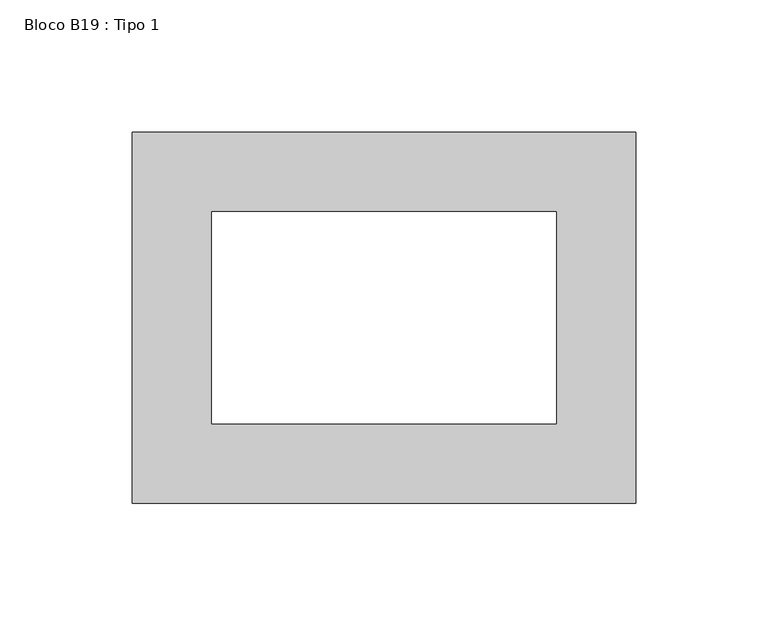
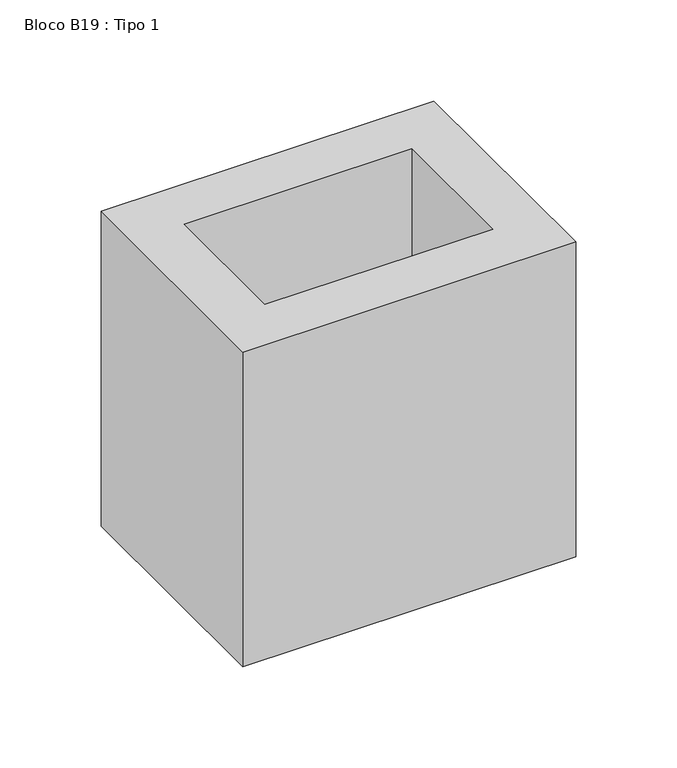
"""IFC4 building model written with IfcOpenShell, lengths in millimetres: proxy geometry, Bloco B19 : Tipo 1."""

from ifc_helpers import new_model, si_unit, origin, origin_with_axes, place, context, project, spatial, polyline, outline, extrude, source, transform, mapped, element, save


def bloco_b19_tipo_1_1abb6ed9(model_context):
    return source(origin(), model_context, "Body", "SweptSolid", [
        extrude(outline(polyline([(190.0, 140.0), (190.0, 0.0), (0.0, 0.0), (0.0, 140.0), (190.0, 140.0)]), holes=[polyline([(30.0, 110.0), (30.0, 30.0), (160.0, 30.0), (160.0, 110.0), (30.0, 110.0)])]), origin_with_axes(), (0.0, 0.0, 1.0), 190.0),
    ])


if __name__ == "__main__":
    model = new_model("IFC4")
    model_context = context("Model", 3, world=origin())
    ifc_project = project(units=[si_unit("LENGTHUNIT", "METRE", prefix="MILLI")], contexts=[model_context])
    site = spatial("IfcSite", under=ifc_project)
    building = spatial("IfcBuilding", under=site)
    placement = place(None, origin())
    bloco_b19_tipo_1_shape = bloco_b19_tipo_1_1abb6ed9(model_context)
    element("IfcBuildingElementProxy", 1, Name="Bloco B19 : Tipo 1", ObjectType="Bloco B19 : Tipo 1", at=placement, inside=building, context=model_context, shape_type="MappedRepresentation", body=[
        mapped(bloco_b19_tipo_1_shape, transform((0.0, 0.0, 0.0), x_axis=(1.0, 0.0, 0.0), y_axis=(0.0, 1.0, 0.0), z_axis=(0.0, 0.0, 1.0))),
    ])
    save(model, "model.ifc")

# Revit data of these elements
# Type "Bloco B19 : Tipo 1"
#   SINAPI = ""
#   Assembly Code = ""
